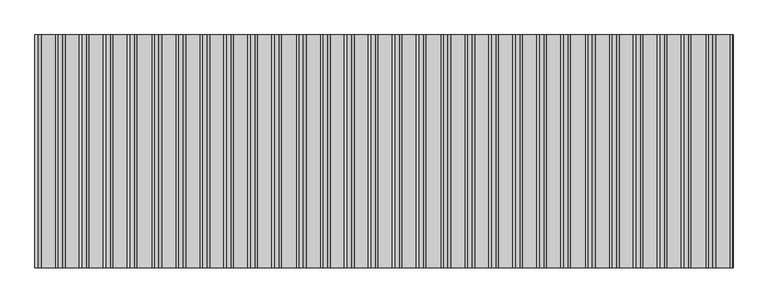
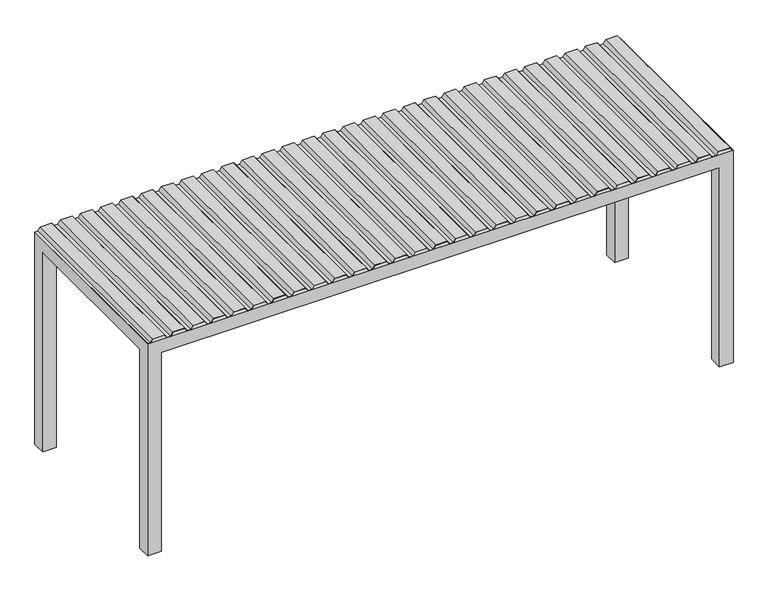
"""IFC4 building model written with IfcOpenShell, lengths in millimetres: proxy geometry, NLRS_90_GM_WPB_fietsenstalling-open_gen_rsf : fietsenstalling bxd 6000x2000mm."""

import ifcopenshell
import ifcopenshell.guid

model = None  # the IFC model being written
_history = None  # IfcOwnerHistory: only IFC2X3 demands one
_inside = {}  # id of a spatial element -> (the spatial element, [elements in it])
_under = {}  # id of a project, library or spatial element -> (it, [spatial elements below it])
_declared = {}  # id of a project -> (the project, [libraries it declares])
_typed = {}  # id of a type object -> (the type object, [elements of that type])
_made_of = {}  # id of a material, layer set ... -> (it, [elements and type objects made of it])


def new_model(schema):
    """Start an empty IFC model of exactly this schema.

    Asked for "IFC4X3", IfcOpenShell would pick the latest addendum, in which some entities
    have other attributes; the version numbers below select the first issue.
    IFC2X3 requires an IfcOwnerHistory on every rooted entity: one is made here for all.
    """
    global model, _history
    if schema == "IFC4X3":
        model = ifcopenshell.file(schema_version=(4, 3, 0, 0))
    else:
        model = ifcopenshell.file(schema=schema)
    _inside.clear()
    _under.clear()
    _declared.clear()
    _typed.clear()
    _made_of.clear()
    _history = None
    if model.schema == "IFC2X3":
        org = make("IfcOrganization", Name="unknown")
        user = make(
            "IfcPersonAndOrganization",
            ThePerson=make("IfcPerson", FamilyName="unknown"),
            TheOrganization=org,
        )
        app = make(
            "IfcApplication",
            ApplicationDeveloper=org,
            Version="unknown",
            ApplicationFullName="unknown",
            ApplicationIdentifier="unknown",
        )
        _history = make(
            "IfcOwnerHistory",
            OwningUser=user,
            OwningApplication=app,
            ChangeAction="ADDED",
            CreationDate=0,
        )
    return model


def make(cls, **values):
    """One entity of the class cls with the attributes given. An attribute that is None is left unset."""
    return model.create_entity(
        cls, **{name: value for name, value in values.items() if value is not None}
    )


def rooted(cls, **values):
    """An entity with a GlobalId (a new one), such as an element, a storey or a relation."""
    return make(cls, GlobalId=ifcopenshell.guid.new(), OwnerHistory=_history, **values)


def si_unit(unit_type, name, prefix=None):
    """IfcSIUnit, for example si_unit("LENGTHUNIT", "METRE", prefix="MILLI")."""
    return make("IfcSIUnit", UnitType=unit_type, Prefix=prefix, Name=name)


def assignment(units):
    """IfcUnitAssignment: the units of a project."""
    return None if units is None else make("IfcUnitAssignment", Units=units)


def point(xyz):
    """IfcCartesianPoint."""
    return None if xyz is None else make("IfcCartesianPoint", Coordinates=xyz)


def direction(xyz):
    """IfcDirection."""
    return None if xyz is None else make("IfcDirection", DirectionRatios=xyz)


def frame(location, z_axis=None, x_axis=None):
    """IfcAxis2Placement3D, a coordinate frame: its origin and axes. An axis left out is left unset."""
    return make(
        "IfcAxis2Placement3D",
        Location=point(location),
        Axis=direction(z_axis),
        RefDirection=direction(x_axis),
    )


def origin():
    """The frame at (0, 0, 0) with its axes left unset."""
    return frame((0.0, 0.0, 0.0))


def place(relative_to, where):
    """IfcLocalPlacement: puts the frame where relative to a parent placement (None: the world)."""
    return make(
        "IfcLocalPlacement", PlacementRelTo=relative_to, RelativePlacement=where
    )


def context(
    kind, dimensions, precision=None, world=None, true_north=None, identifier=None
):
    """IfcGeometricRepresentationContext, for example the 3D "Model" context."""
    return make(
        "IfcGeometricRepresentationContext",
        ContextIdentifier=identifier,
        ContextType=kind,
        CoordinateSpaceDimension=dimensions,
        Precision=precision,
        WorldCoordinateSystem=world,
        TrueNorth=true_north,
    )


def project(units=None, contexts=None):
    """IfcProject with its units and contexts."""
    return rooted(
        "IfcProject",
        Name="project",
        RepresentationContexts=contexts,
        UnitsInContext=assignment(units),
    )


def spatial(cls, under=None, at=None, **own):
    """A site, building, storey or space (cls), placed at a placement, below another one or the project."""
    s = rooted(cls, ObjectPlacement=at, **own)
    if under is not None:
        _under.setdefault(under.id(), (under, []))[1].append(s)
    return s


def polyline(points):
    """IfcPolyline through the points."""
    return make("IfcPolyline", Points=[point(p) for p in points])


def outline(outer, holes=None, kind="AREA"):
    """IfcArbitraryClosedProfileDef: a profile drawn as a closed curve; with holes, ...WithVoids."""
    if holes is None:
        return make("IfcArbitraryClosedProfileDef", ProfileType=kind, OuterCurve=outer)
    return make(
        "IfcArbitraryProfileDefWithVoids",
        ProfileType=kind,
        OuterCurve=outer,
        InnerCurves=holes,
    )


def extrude(swept, where, along, depth):
    """IfcExtrudedAreaSolid: the profile swept, set in the frame where, extruded along a direction by depth."""
    return make(
        "IfcExtrudedAreaSolid",
        SweptArea=swept,
        Position=where,
        ExtrudedDirection=direction(along),
        Depth=depth,
    )


def faces_of(points, faces, orient=None, outer=None):
    """IfcFace entities. A face is a list of loops; a loop is a list of indices into points, from 0.

    orient and outer hold one flag for each loop. By default every Orientation is true, the
    first loop of a face is its IfcFaceOuterBound and the others are IfcFaceBound.
    """
    made = []
    for i, loops in enumerate(faces):
        bounds = []
        for j, loop in enumerate(loops):
            is_outer = j == 0 if outer is None else outer[i][j]
            bounds.append(
                make(
                    "IfcFaceOuterBound" if is_outer else "IfcFaceBound",
                    Bound=make("IfcPolyLoop", Polygon=[points[k] for k in loop]),
                    Orientation=True if orient is None else orient[i][j],
                )
            )
        made.append(make("IfcFace", Bounds=bounds))
    return made


def faceted_brep(points, faces, orient=None, outer=None, voids=None):
    """IfcFacetedBrep: a solid bounded by flat faces; with voids (closed shells), ...WithVoids."""
    shared = [point(p) for p in points]
    hull = make("IfcClosedShell", CfsFaces=faces_of(shared, faces, orient, outer))
    if voids is None:
        return make("IfcFacetedBrep", Outer=hull)
    return make(
        "IfcFacetedBrepWithVoids",
        Outer=hull,
        Voids=[
            make(cls, CfsFaces=faces_of(shared, fs, o, b)) for cls, fs, o, b in voids
        ],
    )


def shape(context_of_items, identifier, shape_type, items):
    """IfcShapeRepresentation: the items that make up one representation, for example the "Body"."""
    return make(
        "IfcShapeRepresentation",
        ContextOfItems=context_of_items,
        RepresentationIdentifier=identifier,
        RepresentationType=shape_type,
        Items=items,
    )


def source(mapping_origin, context_of_items, identifier, shape_type, items):
    """IfcRepresentationMap: a shape defined once, which mapped items show again and again."""
    return make(
        "IfcRepresentationMap",
        MappingOrigin=mapping_origin,
        MappedRepresentation=shape(context_of_items, identifier, shape_type, items),
    )


def transform(
    local_origin,
    x_axis=None,
    y_axis=None,
    z_axis=None,
    scale=None,
    scale2=None,
    scale3=None,
    uniform=True,
):
    """IfcCartesianTransformationOperator3D, or its non-uniform kind. x_axis, y_axis, z_axis: its Axis1, 2, 3."""
    if uniform:
        return make(
            "IfcCartesianTransformationOperator3D",
            Axis1=direction(x_axis),
            Axis2=direction(y_axis),
            LocalOrigin=point(local_origin),
            Scale=scale,
            Axis3=direction(z_axis),
        )
    return make(
        "IfcCartesianTransformationOperator3DnonUniform",
        Axis1=direction(x_axis),
        Axis2=direction(y_axis),
        LocalOrigin=point(local_origin),
        Scale=scale,
        Axis3=direction(z_axis),
        Scale2=scale2,
        Scale3=scale3,
    )


def mapped(mapping_source, mapping_target):
    """IfcMappedItem: shows the shape of a source again, moved by a transform."""
    return make(
        "IfcMappedItem", MappingSource=mapping_source, MappingTarget=mapping_target
    )


def made_of(thing, what):
    """Note that an element or type object is made of a material, layer set ...; save() writes the relation."""
    if what is not None:
        _made_of.setdefault(what.id(), (what, []))[1].append(thing)
    return thing


def element(
    cls,
    number,
    at=None,
    inside=None,
    cuts=None,
    type_object=None,
    material=None,
    context=None,
    identifier="Body",
    shape_type=None,
    held_by="IfcProductDefinitionShape",
    body=None,
    shapes=None,
    **own,
):
    """One element of the class cls, such as IfcWall. Its Tag is "e" and its number.

    at: its placement. inside: the storey or other place that contains it. cuts: it is an
    opening in that element (IfcRelVoidsElement). A single representation is given by context,
    identifier, shape_type and body (its items); several are given by shapes. held_by: the class
    of the entity that holds the representations. save() writes the other relations.
    """
    e = rooted(cls, Tag="e%d" % number, ObjectPlacement=at, **own)
    if body is not None:
        shapes = [shape(context, identifier, shape_type, body)]
    if shapes is not None:
        e.Representation = make(held_by, Representations=shapes)
    if inside is not None:
        _inside.setdefault(inside.id(), (inside, []))[1].append(e)
    if cuts is not None:
        rooted(
            "IfcRelVoidsElement", RelatingBuildingElement=cuts, RelatedOpeningElement=e
        )
    if type_object is not None:
        _typed.setdefault(type_object.id(), (type_object, []))[1].append(e)
    return made_of(e, material)


def aggregate(whole, parts):
    """IfcRelAggregates: a whole, such as a stair, and the parts it consists of."""
    return rooted("IfcRelAggregates", RelatingObject=whole, RelatedObjects=parts)


def save(model, path):
    """Write the relations noted so far, then the file.

    IfcRelAggregates (storeys below a building ...), IfcRelContainedInSpatialStructure (elements
    in a storey), IfcRelDefinesByType, IfcRelAssociatesMaterial and IfcRelDeclares: one each for
    every whole, place, type object, material and project.
    """
    for whole, parts in _under.values():
        aggregate(whole, parts)
    for where, things in _inside.values():
        rooted(
            "IfcRelContainedInSpatialStructure",
            RelatedElements=things,
            RelatingStructure=where,
        )
    for kind, things in _typed.values():
        rooted("IfcRelDefinesByType", RelatedObjects=things, RelatingType=kind)
    for what, things in _made_of.values():
        rooted("IfcRelAssociatesMaterial", RelatedObjects=things, RelatingMaterial=what)
    for by, libraries in _declared.values():
        rooted("IfcRelDeclares", RelatingContext=by, RelatedDefinitions=libraries)
    model.write(path)


def generic_models_a46722be(model_context):
    return source(origin(), model_context, "Body", "SolidModel", [
        extrude(outline(polyline([(2335.0, -2946.0022315), (2335.0, -2826.9992824), (2300.0, -2803.0007176), (2300.0, -2763.0007963), (2335.0, -2739.0022315), (2335.0, -2619.9992824), (2300.0, -2596.0007176), (2300.0, -2556.0007963), (2335.0, -2532.0022315), (2335.0, -2412.9992824), (2300.0, -2389.0007176), (2300.0, -2349.0007963), (2335.0, -2325.0022315), (2335.0, -2205.9992824), (2300.0, -2182.0007176), (2300.0, -2142.0007963), (2335.0, -2118.0022315), (2335.0, -1998.9992824), (2300.0, -1975.0007176), (2300.0, -1934.9987283), (2335.0, -1911.0001636), (2335.0, -1791.9972144), (2300.0, -1767.9986497), (2300.0, -1727.9987283), (2335.0, -1704.0001636), (2335.0, -1584.9972144), (2300.0, -1560.9986497), (2300.0, -1520.9987283), (2335.0, -1497.0001636), (2335.0, -1377.9972144), (2300.0, -1353.9986497), (2300.0, -1313.9987283), (2335.0, -1290.0001636), (2335.0, -1170.9972144), (2300.0, -1146.9986497), (2300.0, -1106.9987283), (2335.0, -1083.0001636), (2335.0, -963.9972144), (2300.0, -939.9986497), (2300.0, -899.9966604), (2335.0, -875.9980957), (2335.0, -756.9951465), (2300.0, -732.9965818), (2300.0, -692.9966604), (2335.0, -668.9980957), (2335.0, -549.9951465), (2300.0, -525.9965818), (2300.0, -485.9966604), (2335.0, -461.9980957), (2335.0, -342.9951465), (2300.0, -318.9965818), (2300.0, -278.9966604), (2335.0, -254.9980957), (2335.0, -135.9951465), (2300.0, -111.9965818), (2300.0, -71.9966604), (2335.0, -47.9980957), (2335.0, 71.0048535), (2300.0, 95.0034182), (2300.0, 135.0054075), (2335.0, 159.0039722), (2335.0, 278.0069214), (2300.0, 302.0054861), (2300.0, 342.0054075), (2335.0, 366.0039722), (2335.0, 485.0069214), (2300.0, 509.0054861), (2300.0, 549.0054075), (2335.0, 573.0039722), (2335.0, 692.0069214), (2300.0, 716.0054861), (2300.0, 756.0054075), (2335.0, 780.0039722), (2335.0, 899.0069214), (2300.0, 923.0054861), (2300.0, 963.0054075), (2335.0, 987.0039722), (2335.0, 1106.0069214), (2300.0, 1130.0054861), (2300.0, 1170.0074754), (2335.0, 1194.0060401), (2335.0, 1313.0089893), (2300.0, 1337.007554), (2300.0, 1377.0074754), (2335.0, 1401.0060401), (2335.0, 1520.0089893), (2300.0, 1544.007554), (2300.0, 1584.0074754), (2335.0, 1608.0060401), (2335.0, 1727.0089893), (2300.0, 1751.007554), (2300.0, 1791.0074754), (2335.0, 1815.0060401), (2335.0, 1934.0089893), (2300.0, 1958.007554), (2300.0, 1998.0074754), (2335.0, 2022.0060401), (2335.0, 2141.0089893), (2300.0, 2165.007554), (2300.0, 2205.0095433), (2335.0, 2229.008108), (2335.0, 2348.0110572), (2300.0, 2372.0096219), (2300.0, 2412.0095433), (2335.0, 2436.008108), (2335.0, 2555.0110572), (2300.0, 2579.0096219), (2300.0, 2619.0095433), (2335.0, 2643.008108), (2335.0, 2762.0110572), (2300.0, 2786.0096219), (2300.0, 2826.0095433), (2335.0, 2850.008108), (2335.0, 2969.0110572), (2300.0, 2993.0096219), (2300.0, 3000.0), (2302.0, 3000.0), (2302.0, 2994.0632684), (2337.0, 2970.0647037), (2337.0, 2848.9544615), (2302.0, 2824.9558968), (2302.0, 2787.0632684), (2337.0, 2763.0647037), (2337.0, 2641.9544615), (2302.0, 2617.9558968), (2302.0, 2580.0632684), (2337.0, 2556.0647037), (2337.0, 2434.9544615), (2302.0, 2410.9558968), (2302.0, 2373.0632684), (2337.0, 2349.0647037), (2337.0, 2227.9544615), (2302.0, 2203.9558968), (2302.0, 2166.0612005), (2337.0, 2142.0626358), (2337.0, 2020.9523936), (2302.0, 1996.9538289), (2302.0, 1959.0612005), (2337.0, 1935.0626358), (2337.0, 1813.9523936), (2302.0, 1789.9538289), (2302.0, 1752.0612005), (2337.0, 1728.0626358), (2337.0, 1606.9523936), (2302.0, 1582.9538289), (2302.0, 1545.0612005), (2337.0, 1521.0626358), (2337.0, 1399.9523936), (2302.0, 1375.9538289), (2302.0, 1338.0612005), (2337.0, 1314.0626358), (2337.0, 1192.9523936), (2302.0, 1168.9538289), (2302.0, 1131.0591326), (2337.0, 1107.0605679), (2337.0, 985.9503257), (2302.0, 961.951761), (2302.0, 924.0591326), (2337.0, 900.0605679), (2337.0, 778.9503257), (2302.0, 754.951761), (2302.0, 717.0591326), (2337.0, 693.0605679), (2337.0, 571.9503257), (2302.0, 547.951761), (2302.0, 510.0591326), (2337.0, 486.0605679), (2337.0, 364.9503257), (2302.0, 340.951761), (2302.0, 303.0591326), (2337.0, 279.0605679), (2337.0, 157.9503257), (2302.0, 133.951761), (2302.0, 96.0570647), (2337.0, 72.0585), (2337.0, -49.0517422), (2302.0, -73.0503069), (2302.0, -110.9429353), (2337.0, -134.9415), (2337.0, -256.0517422), (2302.0, -280.0503069), (2302.0, -317.9429353), (2337.0, -341.9415), (2337.0, -463.0517422), (2302.0, -487.0503069), (2302.0, -524.9429353), (2337.0, -548.9415), (2337.0, -670.0517422), (2302.0, -694.0503069), (2302.0, -731.9429353), (2337.0, -755.9415), (2337.0, -877.0517422), (2302.0, -901.0503069), (2302.0, -938.9450032), (2337.0, -962.9435679), (2337.0, -1084.0538101), (2302.0, -1108.0523749), (2302.0, -1145.9450032), (2337.0, -1169.9435679), (2337.0, -1291.0538101), (2302.0, -1315.0523749), (2302.0, -1352.9450032), (2337.0, -1376.9435679), (2337.0, -1498.0538101), (2302.0, -1522.0523749), (2302.0, -1559.9450032), (2337.0, -1583.9435679), (2337.0, -1705.0538101), (2302.0, -1729.0523749), (2302.0, -1766.9450032), (2337.0, -1790.9435679), (2337.0, -1912.0538101), (2302.0, -1936.0523749), (2302.0, -1973.9470711), (2337.0, -1997.9456358), (2337.0, -2119.055878), (2302.0, -2143.0544428), (2302.0, -2180.9470711), (2337.0, -2204.9456358), (2337.0, -2326.055878), (2302.0, -2350.0544428), (2302.0, -2387.9470711), (2337.0, -2411.9456358), (2337.0, -2533.055878), (2302.0, -2557.0544428), (2302.0, -2594.9470711), (2337.0, -2618.9456358), (2337.0, -2740.055878), (2302.0, -2764.0544428), (2302.0, -2801.9470711), (2337.0, -2825.9456358), (2337.0, -2947.055878), (2302.0, -2971.0544428), (2302.0, -3000.0), (2300.0, -3000.0), (2300.0, -2970.0007963), (2335.0, -2946.0022315)])), frame((0.0, -1000.0, 0.0), z_axis=(0.0, 1.0, 0.0), x_axis=(0.0, 0.0, 1.0)), (0.0, 0.0, 1.0), 2000.0),
        faceted_brep([(-2860.0, -1000.0, 0.0), (-3000.0, -1000.0, 0.0), (-3000.0, -860.0, 0.0), (-2860.0, -860.0, 0.0), (-2860.0, 860.0, 0.0), (-3000.0, 860.0, 0.0), (-3000.0, 1000.0, 0.0), (-2860.0, 1000.0, 0.0), (3000.0, -1000.0, 0.0), (2860.0, -1000.0, 0.0), (2860.0, -860.0, 0.0), (3000.0, -860.0, 0.0), (3000.0, 860.0, 0.0), (2860.0, 860.0, 0.0), (2860.0, 1000.0, 0.0), (3000.0, 1000.0, 0.0), (-2860.0, -1000.0, 2160.0), (2860.0, -1000.0, 2160.0), (3000.0, -1000.0, 2300.0), (-3000.0, -1000.0, 2300.0), (-3000.0, 1000.0, 2300.0), (-3000.0, 860.0, 2160.0), (-3000.0, -860.0, 2160.0), (-2860.0, -860.0, 2160.0), (-2860.0, 860.0, 2160.0), (3000.0, 1000.0, 2300.0), (2860.0, 1000.0, 2160.0), (-2860.0, 1000.0, 2160.0), (2860.0, -860.0, 2160.0), (3000.0, -860.0, 2160.0), (3000.0, 860.0, 2160.0), (2860.0, 860.0, 2160.0), (2860.0, -860.0, 2300.0), (-2860.0, -860.0, 2300.0), (-2860.0, 860.0, 2300.0), (2860.0, 860.0, 2300.0), (2860.0, 860.0, 2223.0), (2860.0, -860.0, 2223.0), (-2860.0, 860.0, 2223.0), (-2860.0, -860.0, 2223.0)], [[[0, 1, 2, 3]], [[4, 5, 6, 7]], [[8, 9, 10, 11]], [[12, 13, 14, 15]], [[0, 16, 17, 9, 8, 18, 19, 1]], [[19, 20, 6, 5, 21, 22, 2, 1]], [[2, 22, 23, 3]], [[3, 23, 16, 0]], [[4, 24, 21, 5]], [[20, 25, 15, 14, 26, 27, 7, 6]], [[7, 27, 24, 4]], [[9, 17, 28, 10]], [[10, 28, 29, 11]], [[11, 29, 30, 12, 15, 25, 18, 8]], [[12, 30, 31, 13]], [[13, 31, 26, 14]], [[18, 25, 20, 19], [32, 33, 34, 35]], [[23, 22, 21, 24]], [[24, 27, 26, 31]], [[28, 17, 16, 23]], [[31, 30, 29, 28]], [[35, 36, 31, 28, 37, 32]], [[34, 38, 24, 31, 36, 35]], [[33, 39, 23, 24, 38, 34]], [[32, 37, 28, 23, 39, 33]]]),
    ])


if __name__ == "__main__":
    model = new_model("IFC4")
    model_context = context("Model", 3, world=origin())
    ifc_project = project(units=[si_unit("LENGTHUNIT", "METRE", prefix="MILLI")], contexts=[model_context])
    site = spatial("IfcSite", under=ifc_project)
    building = spatial("IfcBuilding", under=site)
    placement = place(None, origin())
    generic_models_shape = generic_models_a46722be(model_context)
    element("IfcBuildingElementProxy", 1, Name="NLRS_90_GM_WPB_fietsenstalling-open_gen_rsf : fietsenstalling bxd 6000x2000mm", ObjectType="NLRS_90_GM_WPB_fietsenstalling-open_gen_rsf : fietsenstalling bxd 6000x2000mm", at=placement, inside=building, context=model_context, shape_type="MappedRepresentation", body=[
        mapped(generic_models_shape, transform((0.0, 0.0, 0.0), x_axis=(1.0, 0.0, 0.0), y_axis=(0.0, 1.0, 0.0), z_axis=(0.0, 0.0, 1.0))),
    ])
    save(model, "model.ifc")

# Revit data of these elements
# Type "NLRS_90_GM_WPB_fietsenstalling-open_gen_rsf : fietsenstalling bxd 6000x2000mm"
#   Type IFC Predefined Type = "USERDEFINED"
#   Export Type to IFC As = "IfcGeographicElementType"
#   Type IfcGUID = "1jnPA0m7n0IPwpoVFqywHL"
#   IfcName[Type] = "fietsenstalling bxd 6000x2000mm"
#   IfcDescription[Type] = "fietsenstalling open bxdxh 6000x2000x2300mm"
#   IfcObjectType[Type] = "BICYCLE_STORAGE"
#   IfcExportAs[Type] = "IfcGeographicElementType"
#   IfcExportType[Type] = "USERDEFINED"
#   NLRS_C_omschrijving_01 [instance default] = "dak"
#   NLRS_C_omschrijving [instance default] = "constructie"
#   NLRS_C_materiaal_afwerking_01 [instance default] = ""
#   NLRS_C_materiaal_afwerking [instance default] = ""
#   Model = "generiek"
#   Manufacturer = "generiek"
#   Description = "fietsenstalling open bxdxh 6000x2000x2300mm"
#   Assembly Code = "90.22"
#   constructie_dikte = 140.00 mm
#   NLRS_S_gewicht [instance default] = 0.00 kg
#   NLRS_C_oppervlakte = 12.00 m²
#   NLRS_C_hoogte = 2300.00 mm
#   NLRS_C_diepte = 2000.00 mm
#   NLRS_C_breedte = 6000.00 mm
#   Default Elevation = 1219.20 mm
#   NLRS_C_buiten [instance default] = yes
#   NLRS_C_materiaal_01 = none
#   NLRS_C_materiaal = none
#   URL = ""
